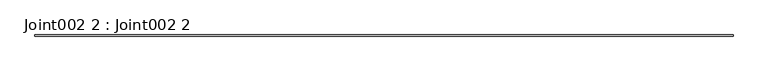
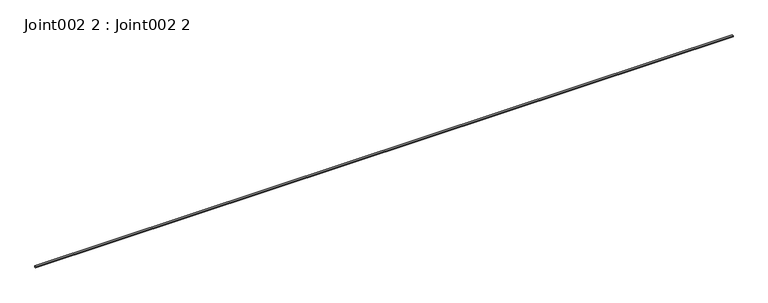
"""IFC4 building model written with IfcOpenShell, lengths in millimetres: proxy geometry, Joint002 2 : Joint002 2."""

from ifc_helpers import new_model, si_unit, point, frame, frame_2d, origin, place, context, project, spatial, polyline, circle_curve, trimmed, segment, composite_curve, outline, extrude, source, transform, mapped, element, save


def joint002_2_joint002_2_1a41533e(model_context):
    return source(origin(), model_context, "Body", "SweptSolid", [
        extrude(outline(composite_curve([segment(polyline([(9718.4918386, 37509.421875), (9718.4918386, 37513.3398437)]), True, "CONTINUOUS"), segment(trimmed(circle_curve(frame_2d((9720.0901706, 37518.5117187)), 5.4132205), [point((9718.4918386, 37513.3398437))], [point((9721.6885026, 37513.3398437))], True, "CARTESIAN"), True, "CONTINUOUS"), segment(polyline([(9721.6885026, 37513.3398437), (9721.6885026, 37509.421875)]), True, "CONTINUOUS"), segment(trimmed(circle_curve(frame_2d((9720.0901706, 37514.59375)), 5.4132205), [point((9721.6885026, 37509.421875))], [point((9718.4918386, 37509.421875))], False, "CARTESIAN"), True, "CONTINUOUS")], self_intersect=False)), frame((3694.2883192, 0.0, 0.0), z_axis=(1.0, 0.0, 0.0), x_axis=(0.0, 1.0, 0.0)), (0.0, 0.0, 1.0), 2000.0),
    ])


if __name__ == "__main__":
    model = new_model("IFC4")
    model_context = context("Model", 3, world=origin())
    ifc_project = project(units=[si_unit("LENGTHUNIT", "METRE", prefix="MILLI")], contexts=[model_context])
    site = spatial("IfcSite", under=ifc_project)
    building = spatial("IfcBuilding", under=site)
    placement = place(None, origin())
    joint002_2_joint002_2_shape = joint002_2_joint002_2_1a41533e(model_context)
    element("IfcBuildingElementProxy", 1, Name="Joint002 2 : Joint002 2", ObjectType="Joint002 2 : Joint002 2", at=placement, inside=building, context=model_context, shape_type="MappedRepresentation", body=[
        mapped(joint002_2_joint002_2_shape, transform((0.0, 0.0, 0.0), x_axis=(1.0, 0.0, 0.0), y_axis=(0.0, 1.0, 0.0), z_axis=(0.0, 0.0, 1.0))),
    ])
    save(model, "model.ifc")

# Revit data of these elements
# Type "Joint002 2 : Joint002 2"
#   NameOverride = "Joint002"
# Element 1 (IfcBuildingElementProxy, "Joint002 2 : Joint002 2")
#   Materials on its faces: "SEALANT JOINT"
# Materials
#   "SEALANT JOINT": class "Unassigned", colour RGB 142 225 148, transparency 0
